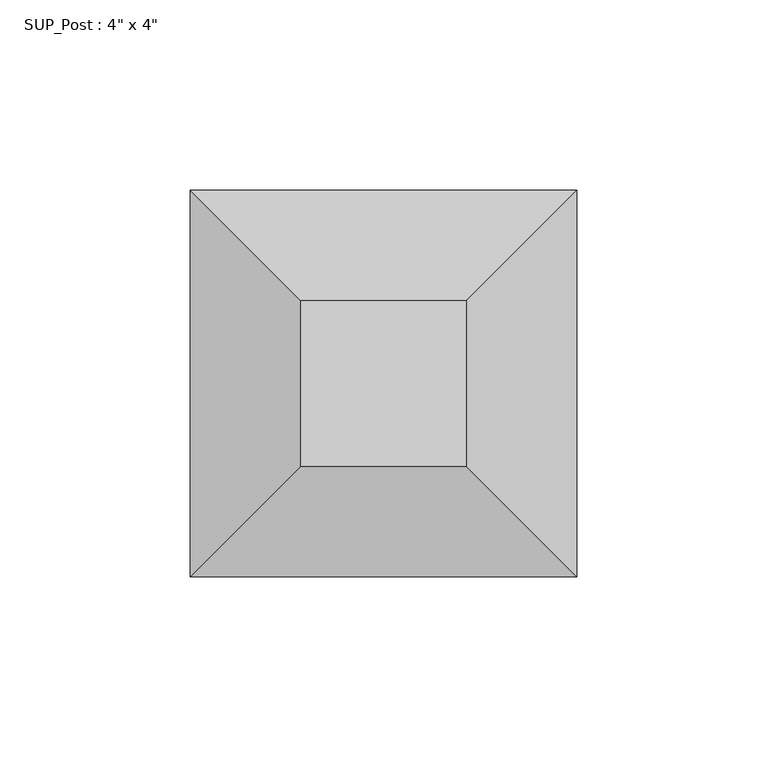
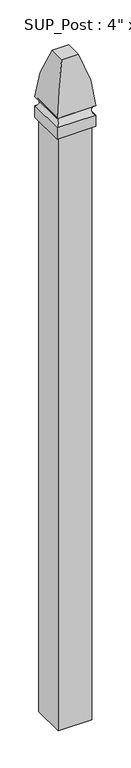
"""IFC4 building model written with IfcOpenShell, lengths in millimetres: proxy geometry."""

from ifc_helpers import new_model, si_unit, frame, origin, place, context, project, spatial, polyline, ellipse_curve, outline, extrude, source, transform, mapped, element, save
from ifc_brep_helpers import plane_surface, cylinder_surface, revolved_surface, advanced_brep


def proxy_fa72a640(model_context):
    return source(origin(), model_context, "Body", "SolidModel", [
        extrude(outline(polyline([(44.45, 107.95), (44.45, 19.05), (-44.45, 19.05), (-44.45, 107.95), (44.45, 107.95)])), frame((0.0, 0.0, -228.6), z_axis=(0.0, 0.0, 1.0), x_axis=(1.0, 0.0, 0.0)), (0.0, 0.0, 1.0), 1676.4),
        advanced_brep(
        [(44.45, 19.05, 1428.75), (44.45, 19.05, 1447.8), (44.45, 107.95, 1447.8), (44.45, 107.95, 1428.75), (50.8, 12.7, 1460.5), (50.8, 12.7, 1428.75), (50.8, 114.3, 1428.75), (50.8, 114.3, 1460.5), (-44.45, 107.95, 1447.8), (-44.45, 107.95, 1428.75), (-50.8, 114.3, 1428.75), (-50.8, 114.3, 1460.5), (-44.45, 19.05, 1447.8), (-44.45, 19.05, 1428.75), (-50.8, 12.7, 1428.75), (-50.8, 12.7, 1460.5), (21.7547368, 85.2547368, 1622.5472198), (-21.7547368, 85.2547368, 1622.5472198), (-21.7547368, 41.7452632, 1622.5472198), (21.7547368, 41.7452632, 1622.5472198), (50.8, 114.3, 1485.9), (50.8, 12.7, 1485.9), (-50.8, 114.3, 1485.9), (-50.8, 12.7, 1485.9)],
        [
            (0, 1),
            (1, 2),
            (2, 3),
            (3, 0),
            (4, 5),
            (5, 6),
            (6, 7),
            (7, 4),
            (2, 8),
            (8, 9),
            (9, 3),
            (6, 10),
            (10, 11),
            (11, 7),
            (8, 12),
            (12, 13),
            (13, 9),
            (10, 14),
            (14, 15),
            (15, 11),
            (0, 13),
            (12, 1),
            (5, 14),
            (4, 15),
            (16, 17),
            (17, 18),
            (18, 19),
            (19, 16),
            (7, 20, ellipse_curve(frame((57.3454302, 120.8454302, 1473.2), z_axis=(-0.7071067811865475, 0.7071067811865475, 0.0), x_axis=(0.7071067811865474, 0.7071067811865476, 0.0)), 20.2055763, 14.2875)),
            (20, 21),
            (21, 4, ellipse_curve(frame((57.3454302, 6.1545698, 1473.2), z_axis=(-0.7071067811865475, -0.7071067811865475, 0.0), x_axis=(-0.7071067811865474, 0.7071067811865476, 0.0)), 20.2055763, 14.2875)),
            (19, 21, ellipse_curve(frame((-351.3440328, 414.8440328, 1471.8321377), z_axis=(0.7071067811865475, 0.7071067811865475, 0.0), x_axis=(0.7071067811865474, -0.7071067811865476, 0.0)), 569.065423, 402.3900195)),
            (20, 16, ellipse_curve(frame((-351.3440328, -287.8440328, 1471.8321377), z_axis=(0.7071067811865475, -0.7071067811865475, 0.0), x_axis=(-0.7071067811865474, -0.7071067811865476, 0.0)), 569.065423, 402.3900195)),
            (11, 22, ellipse_curve(frame((-57.3454302, 120.8454302, 1473.2), z_axis=(-0.7071067811865475, -0.7071067811865475, 0.0), x_axis=(-0.7071067811865476, 0.7071067811865474, 0.0)), 20.2055763, 14.2875)),
            (22, 20),
            (22, 17, ellipse_curve(frame((351.3440328, -287.8440328, 1471.8321377), z_axis=(0.7071067811865475, 0.7071067811865475, 0.0), x_axis=(0.7071067811865476, -0.7071067811865474, 0.0)), 569.065423, 402.3900195)),
            (15, 23, ellipse_curve(frame((-57.3454302, 6.1545698, 1473.2), z_axis=(0.7071067811865475, -0.7071067811865475, 0.0), x_axis=(-0.7071067811865474, -0.7071067811865476, 0.0)), 20.2055763, 14.2875)),
            (23, 22),
            (23, 18, ellipse_curve(frame((351.3440328, 414.8440328, 1471.8321377), z_axis=(-0.7071067811865475, 0.7071067811865475, 0.0), x_axis=(0.7071067811865474, 0.7071067811865476, 0.0)), 569.065423, 402.3900195)),
            (21, 23),
        ],
        [
            plane_surface(frame((44.45, 19.05, 1447.8), z_axis=(-1.0, 0.0, 0.0), x_axis=(0.0, 1.0, 0.0))),
            plane_surface(frame((50.8, 12.7, 1428.75), z_axis=(1.0, 0.0, 0.0), x_axis=(0.0, 1.0, 0.0))),
            plane_surface(frame((44.45, 107.95, 1447.8), z_axis=(0.0, -1.0, 0.0), x_axis=(-1.0, 0.0, 0.0))),
            plane_surface(frame((50.8, 114.3, 1428.75), z_axis=(0.0, 1.0, 0.0), x_axis=(-1.0, 0.0, 0.0))),
            plane_surface(frame((-44.45, 107.95, 1447.8), z_axis=(1.0, 0.0, 0.0), x_axis=(0.0, -1.0, 0.0))),
            plane_surface(frame((-50.8, 114.3, 1428.75), z_axis=(-1.0, 0.0, 0.0), x_axis=(0.0, -1.0, 0.0))),
            plane_surface(frame((-44.45, 19.05, 1447.8), z_axis=(0.0, 1.0, 0.0), x_axis=(1.0, 0.0, 0.0))),
            plane_surface(frame((-15.4047368, 48.0952632, 1447.8), z_axis=(0.0, 0.0, -1.0), x_axis=(1.0, 0.0, 0.0))),
            plane_surface(frame((-44.45, 19.05, 1428.75), z_axis=(0.0, 0.0, -1.0), x_axis=(1.0, 0.0, 0.0))),
            plane_surface(frame((-50.8, 12.7, 1428.75), z_axis=(0.0, -1.0, 0.0), x_axis=(1.0, 0.0, 0.0))),
            plane_surface(frame((-21.7547368, 41.7452632, 1622.5472198), z_axis=(0.0, 0.0, 1.0), x_axis=(1.0, 0.0, 0.0))),
            revolved_surface(polyline([(43.0579302, 135.1329302195122, 1473.2), (43.0579302, -8.132930219512193, 1473.2)]), (57.3454302, 19.05, 1473.2), (0.0, 1.0, 0.0)),
            cylinder_surface(frame((-351.3440328, 19.05, 1471.8321377), z_axis=(0.0, -1.0, 0.0), x_axis=(-1.0, 0.0, 0.0)), 402.3900195),
            revolved_surface(polyline([(-71.63293021951219, 106.5579302, 1473.2), (71.63293021951219, 106.5579302, 1473.2)]), (44.45, 120.8454302, 1473.2), (-1.0, 0.0, 0.0)),
            cylinder_surface(frame((44.45, -287.8440328, 1471.8321377), z_axis=(1.0, 0.0, 0.0), x_axis=(0.0, -1.0, 0.0)), 402.3900195),
            revolved_surface(polyline([(-43.0579302, -8.13293021951219, 1473.2), (-43.0579302, 135.1329302195122, 1473.2)]), (-57.3454302, 107.95, 1473.2), (0.0, -1.0, 0.0)),
            cylinder_surface(frame((351.3440328, 107.95, 1471.8321377), z_axis=(0.0, 1.0, 0.0), x_axis=(1.0, 0.0, 0.0)), 402.3900195),
            revolved_surface(polyline([(71.63293021951218, 20.4420698, 1473.2), (-71.63293021951219, 20.4420698, 1473.2)]), (-44.45, 6.1545698, 1473.2), (1.0, 0.0, 0.0)),
            cylinder_surface(frame((-44.45, 414.8440328, 1471.8321377), z_axis=(-1.0, 0.0, 0.0), x_axis=(0.0, 1.0, 0.0)), 402.3900195),
        ],
        [
            (0, [[1, 2, 3, 4]]),
            (1, [[5, 6, 7, 8]]),
            (2, [[-3, 9, 10, 11]]),
            (3, [[-7, 12, 13, 14]]),
            (4, [[-10, 15, 16, 17]]),
            (5, [[-13, 18, 19, 20]]),
            (6, [[-1, 21, -16, 22]]),
            (7, [[-2, -22, -15, -9]]),
            (8, [[-6, 23, -18, -12], [-4, -11, -17, -21]]),
            (9, [[-5, 24, -19, -23]]),
            (10, [[25, 26, 27, 28]]),
            (11, [[-8, 29, 30, 31]]),
            (12, [[-28, 32, -30, 33]]),
            (13, [[-14, 34, 35, -29]]),
            (14, [[-25, -33, -35, 36]]),
            (15, [[-20, 37, 38, -34]]),
            (16, [[-26, -36, -38, 39]]),
            (17, [[-24, -31, 40, -37]]),
            (18, [[-27, -39, -40, -32]]),
        ],
    ),
    ])


if __name__ == "__main__":
    model = new_model("IFC4")
    model_context = context("Model", 3, world=origin())
    ifc_project = project(units=[si_unit("LENGTHUNIT", "METRE", prefix="MILLI")], contexts=[model_context])
    site = spatial("IfcSite", under=ifc_project)
    building = spatial("IfcBuilding", under=site)
    placement = place(None, origin())
    proxy_shape = proxy_fa72a640(model_context)
    element("IfcBuildingElementProxy", 1, Name="SUP_Post : 4\" x 4\"", ObjectType="SUP_Post : 4\" x 4\"", at=placement, inside=building, context=model_context, shape_type="MappedRepresentation", body=[
        mapped(proxy_shape, transform((0.0, 0.0, 0.0), x_axis=(1.0, 0.0, 0.0), y_axis=(0.0, 1.0, 0.0), z_axis=(0.0, 0.0, 1.0))),
    ])
    save(model, "model.ifc")

# Revit data of these elements
# Type "SUP_Post : 4\" x 4\""
#   W = 0' - 3 1/2"
#   Post Offset = 0' - 2 1/2"
#   Bottom Extension = 0' - 9"
#   built-in parameter 1152166 = 4.75 (stored number, unit not read)
#   built-in parameter 1152165 [instance default] = 0.25 (stored number, unit not read)
#   D = 0' - 3 1/2"
#   Support Material = Pine
# Element 1 (IfcBuildingElementProxy, "SUP_Post : 4\" x 4\"")
#   built-in parameter 1152165 = 0.208333 (stored number, unit not read)
#   Materials on its faces: "Pine"
# Materials
#   "Pine": class "Wood", colour RGB 229 189 132, transparency 0, Description = "Pinus Echinata", Cost = 0
